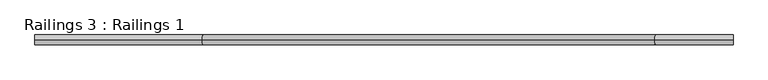
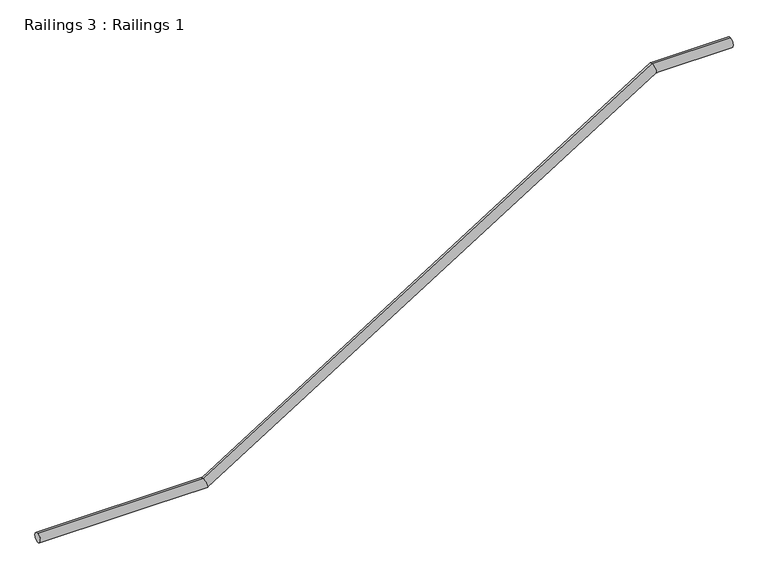
"""IFC4 building model written with IfcOpenShell, lengths in millimetres: railing geometry, Railings 3 : Railings 1."""

import ifcopenshell
import ifcopenshell.guid

model = None  # the IFC model being written
_history = None  # IfcOwnerHistory: only IFC2X3 demands one
_inside = {}  # id of a spatial element -> (the spatial element, [elements in it])
_under = {}  # id of a project, library or spatial element -> (it, [spatial elements below it])
_declared = {}  # id of a project -> (the project, [libraries it declares])
_typed = {}  # id of a type object -> (the type object, [elements of that type])
_made_of = {}  # id of a material, layer set ... -> (it, [elements and type objects made of it])


def new_model(schema):
    """Start an empty IFC model of exactly this schema.

    Asked for "IFC4X3", IfcOpenShell would pick the latest addendum, in which some entities
    have other attributes; the version numbers below select the first issue.
    IFC2X3 requires an IfcOwnerHistory on every rooted entity: one is made here for all.
    """
    global model, _history
    if schema == "IFC4X3":
        model = ifcopenshell.file(schema_version=(4, 3, 0, 0))
    else:
        model = ifcopenshell.file(schema=schema)
    _inside.clear()
    _under.clear()
    _declared.clear()
    _typed.clear()
    _made_of.clear()
    _history = None
    if model.schema == "IFC2X3":
        org = make("IfcOrganization", Name="unknown")
        user = make(
            "IfcPersonAndOrganization",
            ThePerson=make("IfcPerson", FamilyName="unknown"),
            TheOrganization=org,
        )
        app = make(
            "IfcApplication",
            ApplicationDeveloper=org,
            Version="unknown",
            ApplicationFullName="unknown",
            ApplicationIdentifier="unknown",
        )
        _history = make(
            "IfcOwnerHistory",
            OwningUser=user,
            OwningApplication=app,
            ChangeAction="ADDED",
            CreationDate=0,
        )
    return model


def make(cls, **values):
    """One entity of the class cls with the attributes given. An attribute that is None is left unset."""
    return model.create_entity(
        cls, **{name: value for name, value in values.items() if value is not None}
    )


def rooted(cls, **values):
    """An entity with a GlobalId (a new one), such as an element, a storey or a relation."""
    return make(cls, GlobalId=ifcopenshell.guid.new(), OwnerHistory=_history, **values)


def si_unit(unit_type, name, prefix=None):
    """IfcSIUnit, for example si_unit("LENGTHUNIT", "METRE", prefix="MILLI")."""
    return make("IfcSIUnit", UnitType=unit_type, Prefix=prefix, Name=name)


def assignment(units):
    """IfcUnitAssignment: the units of a project."""
    return None if units is None else make("IfcUnitAssignment", Units=units)


def point(xyz):
    """IfcCartesianPoint."""
    return None if xyz is None else make("IfcCartesianPoint", Coordinates=xyz)


def direction(xyz):
    """IfcDirection."""
    return None if xyz is None else make("IfcDirection", DirectionRatios=xyz)


def frame(location, z_axis=None, x_axis=None):
    """IfcAxis2Placement3D, a coordinate frame: its origin and axes. An axis left out is left unset."""
    return make(
        "IfcAxis2Placement3D",
        Location=point(location),
        Axis=direction(z_axis),
        RefDirection=direction(x_axis),
    )


def origin():
    """The frame at (0, 0, 0) with its axes left unset."""
    return frame((0.0, 0.0, 0.0))


def place(relative_to, where):
    """IfcLocalPlacement: puts the frame where relative to a parent placement (None: the world)."""
    return make(
        "IfcLocalPlacement", PlacementRelTo=relative_to, RelativePlacement=where
    )


def context(
    kind, dimensions, precision=None, world=None, true_north=None, identifier=None
):
    """IfcGeometricRepresentationContext, for example the 3D "Model" context."""
    return make(
        "IfcGeometricRepresentationContext",
        ContextIdentifier=identifier,
        ContextType=kind,
        CoordinateSpaceDimension=dimensions,
        Precision=precision,
        WorldCoordinateSystem=world,
        TrueNorth=true_north,
    )


def project(units=None, contexts=None):
    """IfcProject with its units and contexts."""
    return rooted(
        "IfcProject",
        Name="project",
        RepresentationContexts=contexts,
        UnitsInContext=assignment(units),
    )


def spatial(cls, under=None, at=None, **own):
    """A site, building, storey or space (cls), placed at a placement, below another one or the project."""
    s = rooted(cls, ObjectPlacement=at, **own)
    if under is not None:
        _under.setdefault(under.id(), (under, []))[1].append(s)
    return s


def circle_curve(where, radius):
    """IfcCircle in the frame where."""
    return make("IfcCircle", Position=where, Radius=radius)


def ellipse_curve(where, semi_axis1, semi_axis2):
    """IfcEllipse in the frame where."""
    return make(
        "IfcEllipse", Position=where, SemiAxis1=semi_axis1, SemiAxis2=semi_axis2
    )


def shape(context_of_items, identifier, shape_type, items):
    """IfcShapeRepresentation: the items that make up one representation, for example the "Body"."""
    return make(
        "IfcShapeRepresentation",
        ContextOfItems=context_of_items,
        RepresentationIdentifier=identifier,
        RepresentationType=shape_type,
        Items=items,
    )


def source(mapping_origin, context_of_items, identifier, shape_type, items):
    """IfcRepresentationMap: a shape defined once, which mapped items show again and again."""
    return make(
        "IfcRepresentationMap",
        MappingOrigin=mapping_origin,
        MappedRepresentation=shape(context_of_items, identifier, shape_type, items),
    )


def transform(
    local_origin,
    x_axis=None,
    y_axis=None,
    z_axis=None,
    scale=None,
    scale2=None,
    scale3=None,
    uniform=True,
):
    """IfcCartesianTransformationOperator3D, or its non-uniform kind. x_axis, y_axis, z_axis: its Axis1, 2, 3."""
    if uniform:
        return make(
            "IfcCartesianTransformationOperator3D",
            Axis1=direction(x_axis),
            Axis2=direction(y_axis),
            LocalOrigin=point(local_origin),
            Scale=scale,
            Axis3=direction(z_axis),
        )
    return make(
        "IfcCartesianTransformationOperator3DnonUniform",
        Axis1=direction(x_axis),
        Axis2=direction(y_axis),
        LocalOrigin=point(local_origin),
        Scale=scale,
        Axis3=direction(z_axis),
        Scale2=scale2,
        Scale3=scale3,
    )


def mapped(mapping_source, mapping_target):
    """IfcMappedItem: shows the shape of a source again, moved by a transform."""
    return make(
        "IfcMappedItem", MappingSource=mapping_source, MappingTarget=mapping_target
    )


def made_of(thing, what):
    """Note that an element or type object is made of a material, layer set ...; save() writes the relation."""
    if what is not None:
        _made_of.setdefault(what.id(), (what, []))[1].append(thing)
    return thing


def element(
    cls,
    number,
    at=None,
    inside=None,
    cuts=None,
    type_object=None,
    material=None,
    context=None,
    identifier="Body",
    shape_type=None,
    held_by="IfcProductDefinitionShape",
    body=None,
    shapes=None,
    **own,
):
    """One element of the class cls, such as IfcWall. Its Tag is "e" and its number.

    at: its placement. inside: the storey or other place that contains it. cuts: it is an
    opening in that element (IfcRelVoidsElement). A single representation is given by context,
    identifier, shape_type and body (its items); several are given by shapes. held_by: the class
    of the entity that holds the representations. save() writes the other relations.
    """
    e = rooted(cls, Tag="e%d" % number, ObjectPlacement=at, **own)
    if body is not None:
        shapes = [shape(context, identifier, shape_type, body)]
    if shapes is not None:
        e.Representation = make(held_by, Representations=shapes)
    if inside is not None:
        _inside.setdefault(inside.id(), (inside, []))[1].append(e)
    if cuts is not None:
        rooted(
            "IfcRelVoidsElement", RelatingBuildingElement=cuts, RelatedOpeningElement=e
        )
    if type_object is not None:
        _typed.setdefault(type_object.id(), (type_object, []))[1].append(e)
    return made_of(e, material)


def aggregate(whole, parts):
    """IfcRelAggregates: a whole, such as a stair, and the parts it consists of."""
    return rooted("IfcRelAggregates", RelatingObject=whole, RelatedObjects=parts)


def save(model, path):
    """Write the relations noted so far, then the file.

    IfcRelAggregates (storeys below a building ...), IfcRelContainedInSpatialStructure (elements
    in a storey), IfcRelDefinesByType, IfcRelAssociatesMaterial and IfcRelDeclares: one each for
    every whole, place, type object, material and project.
    """
    for whole, parts in _under.values():
        aggregate(whole, parts)
    for where, things in _inside.values():
        rooted(
            "IfcRelContainedInSpatialStructure",
            RelatedElements=things,
            RelatingStructure=where,
        )
    for kind, things in _typed.values():
        rooted("IfcRelDefinesByType", RelatedObjects=things, RelatingType=kind)
    for what, things in _made_of.values():
        rooted("IfcRelAssociatesMaterial", RelatedObjects=things, RelatingMaterial=what)
    for by, libraries in _declared.values():
        rooted("IfcRelDeclares", RelatingContext=by, RelatedDefinitions=libraries)
    model.write(path)


def plane_surface(at):
    """IfcPlane: the flat surface through the origin of the frame at, square to its z axis."""
    return make("IfcPlane", Position=at)


def cylinder_surface(at, radius):
    """IfcCylindricalSurface: all points at the distance radius from the z axis of the frame at."""
    return make("IfcCylindricalSurface", Position=at, Radius=radius)


def advanced_brep(points, edges, surfaces, faces):
    """IfcAdvancedBrep: a solid bounded by faces that lie on surfaces and meet in shared edges.

    An edge is (start, end): straight between two places in points (the first is 0);
    or (start, end, curve); or (start, end, curve, False) where it runs against its curve.
    A face is (place in surfaces, loops), or (place, loops, False) where it looks against
    its surface's normal. A loop lists edges by number (the first is 1), with a minus sign
    where the edge is run from its end to its start. The first loop is the outer one.
    """
    corners = [point(p) for p in points]
    vertices = [make("IfcVertexPoint", VertexGeometry=c) for c in corners]
    made = []
    for start, end, *more in edges:
        made.append(
            make(
                "IfcEdgeCurve",
                EdgeStart=vertices[start],
                EdgeEnd=vertices[end],
                EdgeGeometry=more[0] if more else make("IfcPolyline", Points=[corners[start], corners[end]]),
                SameSense=more[1] if len(more) > 1 else True,
            )
        )
    hull = []
    for where, loops, *sense in faces:
        bounds = []
        for j, loop in enumerate(loops):
            ring = [make("IfcOrientedEdge", EdgeElement=made[abs(k) - 1], Orientation=k > 0) for k in loop]
            bounds.append(
                make(
                    "IfcFaceOuterBound" if j == 0 else "IfcFaceBound",
                    Bound=make("IfcEdgeLoop", EdgeList=ring),
                    Orientation=True,
                )
            )
        hull.append(make("IfcAdvancedFace", Bounds=bounds, FaceSurface=surfaces[where], SameSense=sense[0] if sense else True))
    return make("IfcAdvancedBrep", Outer=make("IfcClosedShell", CfsFaces=hull))


def railings_3_railings_1_cac16bb6(model_context):
    return source(origin(), model_context, "Body", "AdvancedBrep", [
        advanced_brep(
        [(24297.256657, 25764.1906612, 269032.0375), (24297.256657, 25764.1906612, 268993.9375), (27039.9969284, 25764.1906612, 270148.05), (27039.9969284, 25764.1906612, 270109.95), (24952.1721504, 25764.1906612, 269032.0375), (24963.1411635, 25764.1906612, 268993.9375), (26729.7124219, 25764.1906612, 270148.05), (26740.681435, 25764.1906612, 270109.95)],
        [
            (0, 1, circle_curve(frame((24297.256657, 25764.1906612, 269012.9875), z_axis=(-1.0, 0.0, 0.0), x_axis=(0.0, 0.0, -1.0)), 19.05)),
            (1, 0, circle_curve(frame((24297.256657, 25764.1906612, 269012.9875), z_axis=(-1.0, 0.0, 0.0), x_axis=(0.0, 0.0, -1.0)), 19.05)),
            (2, 3, circle_curve(frame((27039.9969284, 25764.1906612, 270129.0), z_axis=(1.0, 0.0, 0.0), x_axis=(0.0, 0.0, -1.0)), 19.05)),
            (3, 2, circle_curve(frame((27039.9969284, 25764.1906612, 270129.0), z_axis=(1.0, 0.0, 0.0), x_axis=(0.0, 0.0, -1.0)), 19.05)),
            (0, 4),
            (4, 5, ellipse_curve(frame((24957.656657, 25764.1906612, 269012.9875), z_axis=(-0.9609670094755169, 0.0, -0.27666298397089845), x_axis=(-0.2766629839708988, 0.0, 0.9609670094755169)), 19.8237815, 19.05)),
            (5, 1),
            (5, 4, ellipse_curve(frame((24957.656657, 25764.1906612, 269012.9875), z_axis=(-0.9609670094755169, 0.0, -0.27666298397089845), x_axis=(-0.2766629839708988, 0.0, 0.9609670094755169)), 19.8237815, 19.05)),
            (4, 6),
            (6, 7, ellipse_curve(frame((26735.1969284, 25764.1906612, 270129.0), z_axis=(-0.9609670094755169, 0.0, -0.27666298397089856), x_axis=(0.27666298397089834, 0.0, -0.960967009475517)), 19.8237815, 19.05)),
            (7, 5),
            (7, 6, ellipse_curve(frame((26735.1969284, 25764.1906612, 270129.0), z_axis=(-0.9609670094755169, 0.0, -0.27666298397089856), x_axis=(0.27666298397089834, 0.0, -0.960967009475517)), 19.8237815, 19.05)),
            (6, 2),
            (3, 7),
        ],
        [
            plane_surface(frame((24297.256657, 25745.1406612, 269012.9875), z_axis=(-1.0, 0.0, 0.0), x_axis=(0.0, -1.0, 0.0))),
            plane_surface(frame((27039.9969284, 25745.1406612, 270129.0), z_axis=(1.0, 0.0, 0.0), x_axis=(0.0, -1.0, 0.0))),
            cylinder_surface(frame((24297.256657, 25764.1906612, 269012.9875), z_axis=(-1.0, 0.0, 0.0), x_axis=(0.0, 0.0, -1.0)), 19.05),
            cylinder_surface(frame((24957.656657, 25764.1906612, 269012.9875), z_axis=(-0.8469151866006367, 0.0, -0.5317280006781745), x_axis=(0.5317280006781745, 0.0, -0.8469151866006367)), 19.05),
            cylinder_surface(frame((26735.1969284, 25764.1906612, 270129.0), z_axis=(-1.0, 0.0, 0.0), x_axis=(0.0, 0.0, -1.0)), 19.05),
        ],
        [
            (0, [[1, 2]]),
            (1, [[3, 4]]),
            (2, [[-1, 5, 6, 7]]),
            (2, [[-2, -7, 8, -5]]),
            (3, [[-6, 9, 10, 11]]),
            (3, [[-8, -11, 12, -9]]),
            (4, [[-10, 13, -4, 14]]),
            (4, [[-12, -14, -3, -13]]),
        ],
    ),
    ])


if __name__ == "__main__":
    model = new_model("IFC4")
    model_context = context("Model", 3, world=origin())
    ifc_project = project(units=[si_unit("LENGTHUNIT", "METRE", prefix="MILLI")], contexts=[model_context])
    site = spatial("IfcSite", under=ifc_project)
    building = spatial("IfcBuilding", under=site)
    placement = place(None, origin())
    railings_3_railings_1_shape = railings_3_railings_1_cac16bb6(model_context)
    element("IfcRailing", 1, ObjectType="Railings 3 : Railings 1", at=placement, inside=building, context=model_context, shape_type="MappedRepresentation", body=[
        mapped(railings_3_railings_1_shape, transform((0.0, 0.0, 0.0), x_axis=(1.0, 0.0, 0.0), y_axis=(0.0, 1.0, 0.0), z_axis=(0.0, 0.0, 1.0))),
    ])
    save(model, "model.ifc")

# Revit data of these elements
# Element 1 (IfcRailing, "Railings 3 : Railings 1")
#   Materials on its faces: "ALUM. RAILING"
# Materials
#   "ALUM. RAILING": class "Generic", colour RGB 255 255 255, transparency 0, Cost = 0
